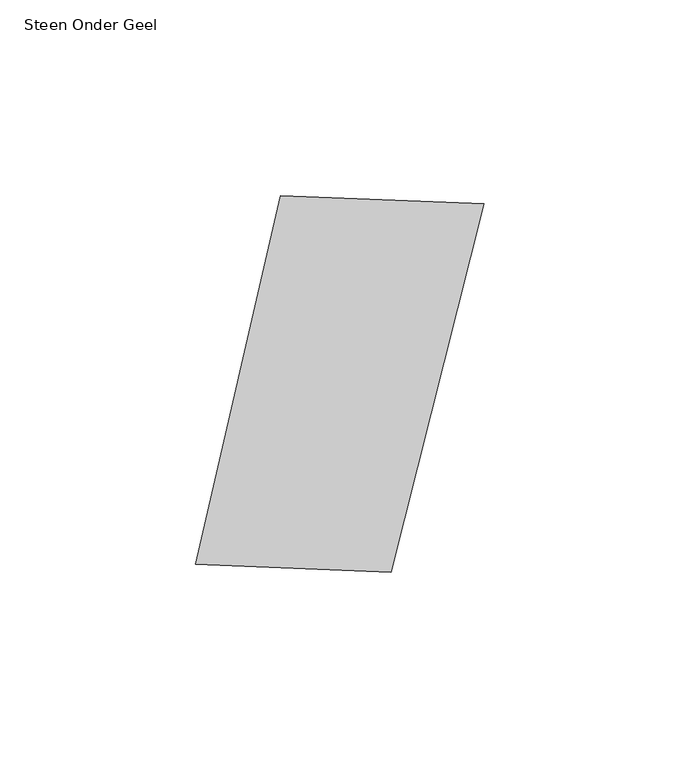
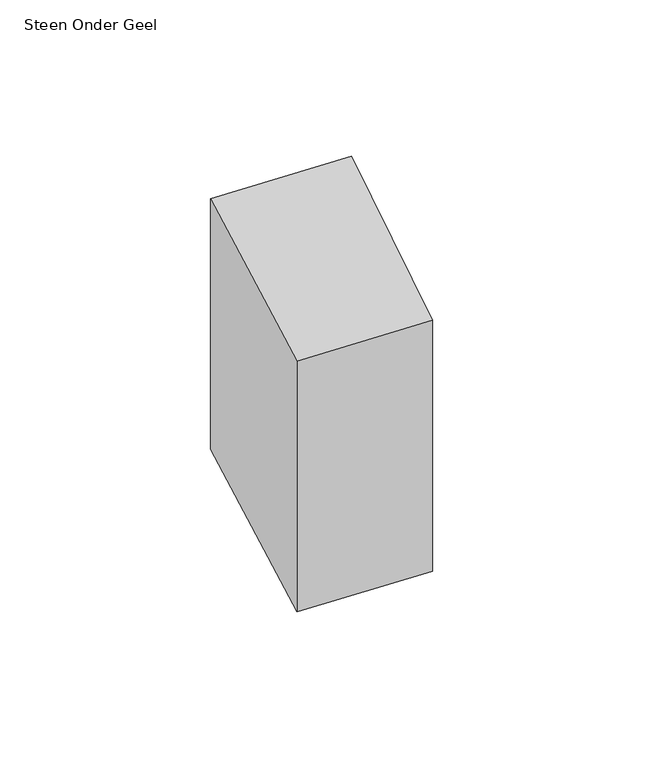
"""IFC4 building model written with IfcOpenShell, lengths in millimetres: proxy geometry, 00_GMA_steen_versie_4 : Steen Onder Geel."""

from ifc_helpers import new_model, si_unit, origin, origin_with_axes, place, context, project, spatial, polyline, outline, extrude, source, transform, mapped, element, save


def steen_onder_geel_1bf8f844(model_context):
    return source(origin(), model_context, "Body", "SweptSolid", [
        extrude(outline(polyline([(111.8862899, 113.4840535), (87.9992869, 19.2623558), (38.0397393, 21.273229), (59.8102837, 115.5625234), (111.8862899, 113.4840535)])), origin_with_axes(), (0.0, 0.0, 1.0), 100.0),
    ])


if __name__ == "__main__":
    model = new_model("IFC4")
    model_context = context("Model", 3, world=origin())
    ifc_project = project(units=[si_unit("LENGTHUNIT", "METRE", prefix="MILLI")], contexts=[model_context])
    site = spatial("IfcSite", under=ifc_project)
    building = spatial("IfcBuilding", under=site)
    placement = place(None, origin())
    steen_onder_geel_shape = steen_onder_geel_1bf8f844(model_context)
    element("IfcBuildingElementProxy", 1, Name="00_GMA_steen_versie_4 : Steen Onder Geel", ObjectType="00_GMA_steen_versie_4 : Steen Onder Geel", at=placement, inside=building, context=model_context, shape_type="MappedRepresentation", body=[
        mapped(steen_onder_geel_shape, transform((0.0, 0.0, 0.0), x_axis=(1.0, 0.0, 0.0), y_axis=(0.0, 1.0, 0.0), z_axis=(0.0, 0.0, 1.0))),
    ])
    save(model, "model.ifc")

# Revit data of these elements
# Type "00_GMA_steen_versie_4 : Steen Onder Geel"
#   StootVoegHalfBoven [instance default] = 5 mm
#   StootVoegHalf [instance default] = 5 mm
#   StootVoegBreedteOnder = 10 mm
#   StootVoegBreedteBoven = 10 mm
#   Steendikte = 100 mm
#   LintVoegOnderHalf = 0 mm
#   LintVoegOnder = 0 mm
#   LintVoegBovenHalf = 5 mm
#   LintVoegBoven = 10 mm
#   materiaal = 21_steen_geel
#   MateriaalVoeg = none
#   Default Elevation = 0
# Element 1 (IfcBuildingElementProxy, "00_GMA_steen_versie_4 : Steen Onder Geel")
#   Materials on its faces: "21_steen_geel"
# Materials
#   "21_steen_geel": class "Unassigned", colour RGB 202 202 0, transparency 0, Cost = 0
